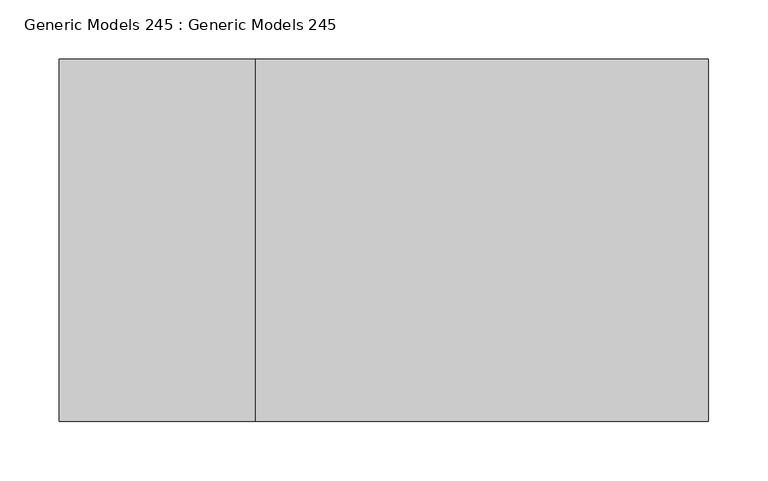
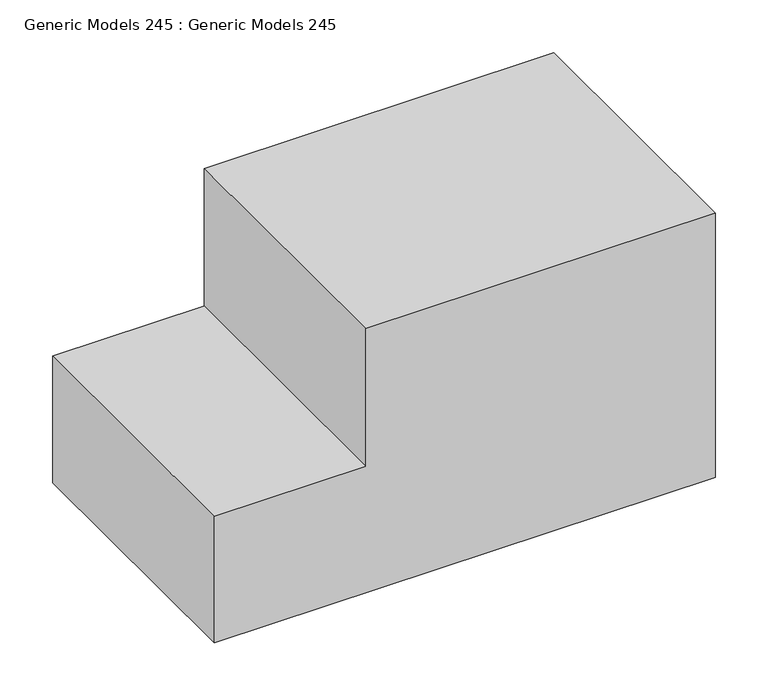
"""IFC4 building model written with IfcOpenShell, lengths in millimetres: proxy geometry, Generic Models 245 : Generic Models 245."""

from ifc_helpers import new_model, si_unit, frame, origin, place, context, project, spatial, polyline, outline, extrude, source, transform, mapped, element, save


def generic_models_245_generic_models_245_5b3b380b(model_context):
    return source(origin(), model_context, "Body", "SweptSolid", [
        extrude(outline(polyline([(123437.396, 1727.0263704), (123291.346, 1727.0263704), (123291.346, 2273.1263704), (123596.146, 2273.1263704), (123596.146, 1892.1263704), (123437.396, 1892.1263704), (123437.396, 1727.0263704)])), frame((0.0, 4260.0872686, 0.0), z_axis=(0.0, 1.0, 0.0), x_axis=(0.0, 0.0, 1.0)), (0.0, 0.0, 1.0), 304.8),
    ])


if __name__ == "__main__":
    model = new_model("IFC4")
    model_context = context("Model", 3, world=origin())
    ifc_project = project(units=[si_unit("LENGTHUNIT", "METRE", prefix="MILLI")], contexts=[model_context])
    site = spatial("IfcSite", under=ifc_project)
    building = spatial("IfcBuilding", under=site)
    placement = place(None, origin())
    generic_models_245_generic_models_245_shape = generic_models_245_generic_models_245_5b3b380b(model_context)
    element("IfcBuildingElementProxy", 1, Name="Generic Models 245 : Generic Models 245", ObjectType="Generic Models 245 : Generic Models 245", at=placement, inside=building, context=model_context, shape_type="MappedRepresentation", body=[
        mapped(generic_models_245_generic_models_245_shape, transform((0.0, 0.0, 0.0), x_axis=(1.0, 0.0, 0.0), y_axis=(0.0, 1.0, 0.0), z_axis=(0.0, 0.0, 1.0))),
    ])
    save(model, "model.ifc")

# Revit data of these elements
# Element 1 (IfcBuildingElementProxy, "Generic Models 245 : Generic Models 245")
#   Materials on its faces: "_CONCRETE SLAB W/ WIRE MESH (SEE STRUCT. DWGS) - SLOPE 1% AWAY FROM BUILDING"
# Materials
#   "_CONCRETE SLAB W/ WIRE MESH (SEE STRUCT. DWGS) - SLOPE 1% AWAY FROM BUILDING": class "Generic", colour RGB 191 191 191, transparency 0, Cost = 0
